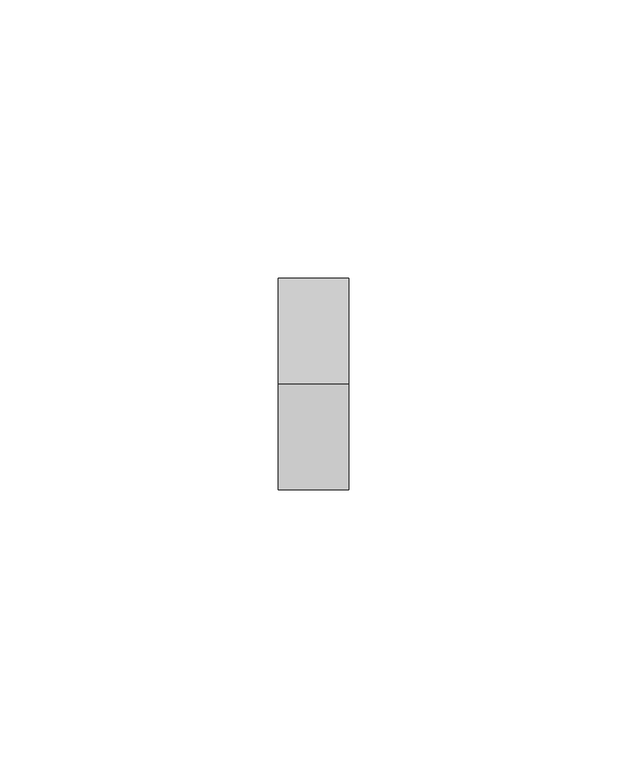
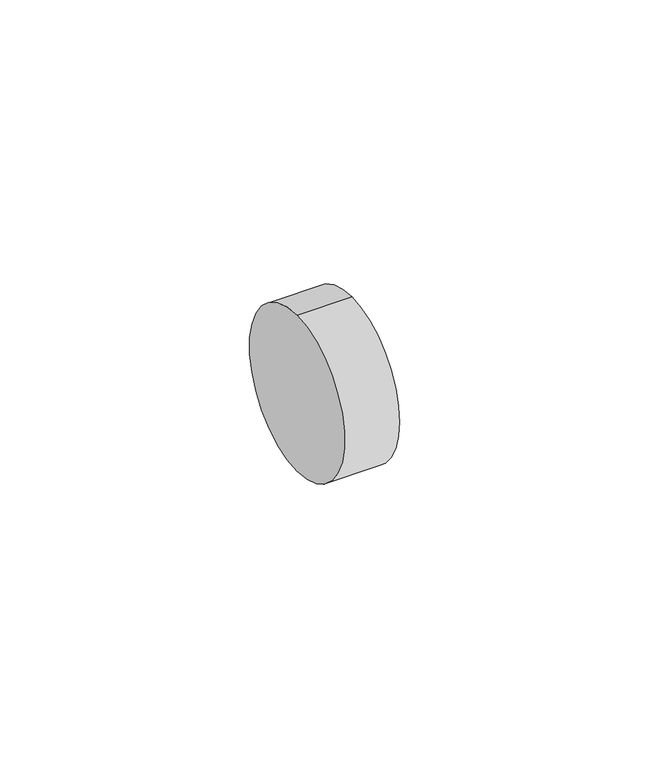
"""IFC4 building model written with IfcOpenShell, lengths in millimetres: proxy geometry, Bolt19:Bolt002:304680 : Bolt19:Bolt002:304680."""

from ifc_helpers import new_model, si_unit, point, frame, frame_2d, origin, place, context, project, spatial, circle_curve, trimmed, segment, composite_curve, outline, extrude, source, transform, mapped, element, save


def generic_models_50c658bf(model_context):
    return source(origin(), model_context, "Body", "SweptSolid", [
        extrude(outline(composite_curve([segment(trimmed(circle_curve(frame_2d((2174.9207483, 40070.0545241)), 19.05), [point((2174.9207483, 40051.0045241))], [point((2174.9207483, 40089.1045241))], False, "CARTESIAN"), True, "CONTINUOUS"), segment(trimmed(circle_curve(frame_2d((2174.9207483, 40070.0545241)), 19.05), [point((2174.9207483, 40089.1045241))], [point((2174.9207483, 40051.0045241))], False, "CARTESIAN"), True, "CONTINUOUS")], self_intersect=False)), frame((15074.8475949, 0.0, 0.0), z_axis=(1.0, 0.0, 0.0), x_axis=(0.0, 1.0, 0.0)), (0.0, 0.0, 1.0), 12.7),
    ])


if __name__ == "__main__":
    model = new_model("IFC4")
    model_context = context("Model", 3, world=origin())
    ifc_project = project(units=[si_unit("LENGTHUNIT", "METRE", prefix="MILLI")], contexts=[model_context])
    site = spatial("IfcSite", under=ifc_project)
    building = spatial("IfcBuilding", under=site)
    placement = place(None, origin())
    generic_models_shape = generic_models_50c658bf(model_context)
    element("IfcBuildingElementProxy", 1, Name="Bolt19:Bolt002:304680 : Bolt19:Bolt002:304680", ObjectType="Bolt19:Bolt002:304680 : Bolt19:Bolt002:304680", at=placement, inside=building, context=model_context, shape_type="MappedRepresentation", body=[
        mapped(generic_models_shape, transform((0.0, 0.0, 0.0), x_axis=(1.0, 0.0, 0.0), y_axis=(0.0, 1.0, 0.0), z_axis=(0.0, 0.0, 1.0))),
    ])
    save(model, "model.ifc")

# Revit data of these elements
# Type "Bolt19:Bolt002:304680 : Bolt19:Bolt002:304680"
#   NameOverride = "Bolt19:Bolt002:304680"
#   ObjectTypeOverride = "Bolt19:Bolt002"
#   Reference = "Bolt002"
#   Category = "Generic Models"
#   Tag = "304680"
# Element 1 (IfcBuildingElementProxy, "Bolt19:Bolt002:304680 : Bolt19:Bolt002:304680")
#   Materials on its faces: "TUBE STEEL STRINGER WELDED TO ANCHORED STEEL PLATE - SEE STRUCT DWGS"
# Materials
#   "TUBE STEEL STRINGER WELDED TO ANCHORED STEEL PLATE - SEE STRUCT DWGS": class "Unassigned", colour RGB 128 128 128, transparency 0, Cost = 0
